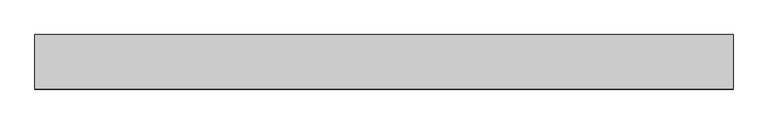
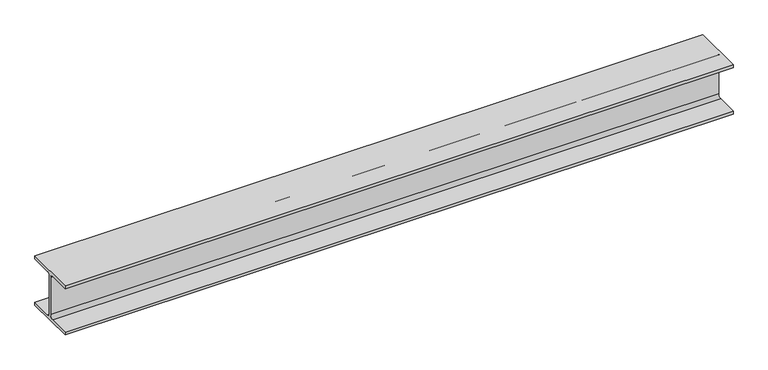
"""IFC4 building model written with IfcOpenShell, lengths in millimetres: beam geometry, 0912_Steel Framing_H-KSD3502 : H_SB_ASB_H-200x200x8x12."""

from ifc_helpers import new_model, si_unit, point, frame, frame_2d, origin, place, context, project, spatial, polyline, circle_curve, trimmed, segment, composite_curve, outline, extrude, source, transform, mapped, element, save


def beam_53ccb7ad(model_context):
    return source(origin(), model_context, "Body", "SweptSolid", [
        extrude(outline(composite_curve([segment(polyline([(100.0, -88.0), (100.0, -100.0), (-100.0, -100.0), (-100.0, -88.0), (-17.0, -88.0)]), True, "CONTINUOUS"), segment(trimmed(circle_curve(frame_2d((-17.0, -75.0)), 13.0), [point((-17.0, -88.0))], [point((-4.0, -75.0))], True, "CARTESIAN"), True, "CONTINUOUS"), segment(polyline([(-4.0, -75.0), (-4.0, 75.0)]), True, "CONTINUOUS"), segment(trimmed(circle_curve(frame_2d((-17.0, 75.0)), 13.0), [point((-4.0, 75.0))], [point((-17.0, 88.0))], True, "CARTESIAN"), True, "CONTINUOUS"), segment(polyline([(-17.0, 88.0), (-100.0, 88.0), (-100.0, 100.0), (100.0, 100.0), (100.0, 88.0), (17.0, 88.0)]), True, "CONTINUOUS"), segment(trimmed(circle_curve(frame_2d((17.0, 75.0)), 13.0), [point((17.0, 88.0))], [point((4.0, 75.0))], True, "CARTESIAN"), True, "CONTINUOUS"), segment(polyline([(4.0, 75.0), (4.0, -75.0)]), True, "CONTINUOUS"), segment(trimmed(circle_curve(frame_2d((17.0, -75.0)), 13.0), [point((4.0, -75.0))], [point((17.0, -88.0))], True, "CARTESIAN"), True, "CONTINUOUS"), segment(polyline([(17.0, -88.0), (100.0, -88.0)]), True, "CONTINUOUS")], self_intersect=False)), frame((-1157.5342344, 0.0, 0.0), z_axis=(1.0, 0.0, 0.0), x_axis=(0.0, 1.0, 0.0)), (0.0, 0.0, 1.0), 2557.991316),
    ])


if __name__ == "__main__":
    model = new_model("IFC4")
    model_context = context("Model", 3, world=origin())
    ifc_project = project(units=[si_unit("LENGTHUNIT", "METRE", prefix="MILLI")], contexts=[model_context])
    site = spatial("IfcSite", under=ifc_project)
    building = spatial("IfcBuilding", under=site)
    placement = place(None, origin())
    beam_shape = beam_53ccb7ad(model_context)
    element("IfcBeam", 1, ObjectType="0912_Steel Framing_H-KSD3502 : H_SB_ASB_H-200x200x8x12", at=placement, inside=building, context=model_context, shape_type="MappedRepresentation", body=[
        mapped(beam_shape, transform((0.0, 0.0, 0.0), x_axis=(1.0, 0.0, 0.0), y_axis=(0.0, 1.0, 0.0), z_axis=(0.0, 0.0, 1.0))),
    ])
    save(model, "model.ifc")

# Revit data of these elements
# Type "0912_Steel Framing_H-KSD3502 : H_SB_ASB_H-200x200x8x12"
#   H_WM Code_1 = "S01AA002-00001 | Main Steel Structure Fabrication Work | Shelter/Building | Medium Steel - Standard (90KG/M>Weight≥30KG/M) | Material: (   )"
#   H_WM Code_2 = "S03AA028-00001 | Main Steel Structure Erection Work | Shelter/Building | Medium Steel (90KG/M>Weight≥30KG/M) | Material: (   )"
#   H_WM Code_3 = "S01AA010-00001 | Main Steel Structure Fabrication Work | Shelter/Building | Steel Painting/Coating | for Non-Fireproofed Steel Surface, Surface Preparation, Primer, Second & Final Coat | Material: (   )"
#   H_Q'ty Cal Type Tag = "SB-Q2"
#   Width = 20.0 cm
#   Web Thickness = 0.8 cm
#   Web Fillet = 1.3 cm
#   Warping Constant = 141000.0 cm⁶
#   W = 0
#   Torsional Moment of Inertia = 26.2485 cm⁴
#   Section Area = 63.53 cm²
#   Plastic Modulus weak axis = 244.0 cm³
#   Plastic Modulus strong axis = 525.0 cm³
#   Perimeter = 1.16 m²/m
#   Nominal Weight = 49.90 kgf/m
#   Moment of Inertia weak axis = 1600.00 cm⁴
#   Moment of Inertia strong axis = 4720.00 cm⁴
#   Height = 20.0 cm
#   Flange Thickness = 1.2 cm
#   Elastic Modulus weak axis = 160.0 cm³
#   Elastic Modulus strong axis = 472.0 cm³
#   Centroid Vertical = 10.0 cm
#   Centroid Horizontal = 10.0 cm
#   Ix = 47200000
#   Length [instance default] = 1.5240 m
#   Zx = 525000
#   b = 0.2000 m
#   h = 0.2000 m
#   r = 0.0130 m
#   s = 0.0080 m
#   t = 0.0120 m
#   A = 0.006353 m²
#   Structural Material [instance default] = Steel, 45-345
#   Assembly Code = ""
# Element 1 (IfcBeam, "0912_Steel Framing_H-KSD3502 : H_SB_ASB_H-200x200x8x12")
#   Structural Material = none
# Materials
#   "Steel, 45-345": class "Metal", colour RGB 189 187 185, transparency 0, Description = "Steel 345 MPa", Cost = 0
